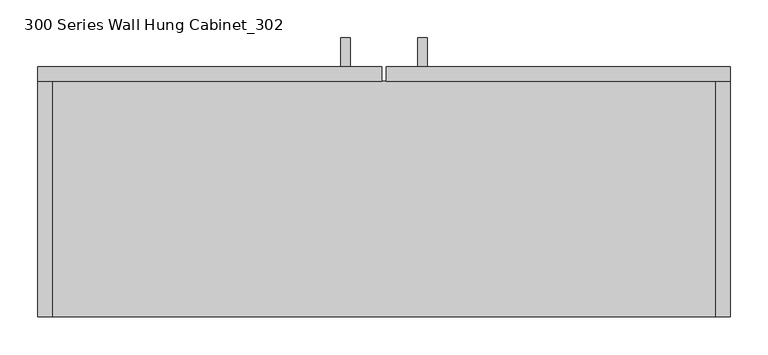
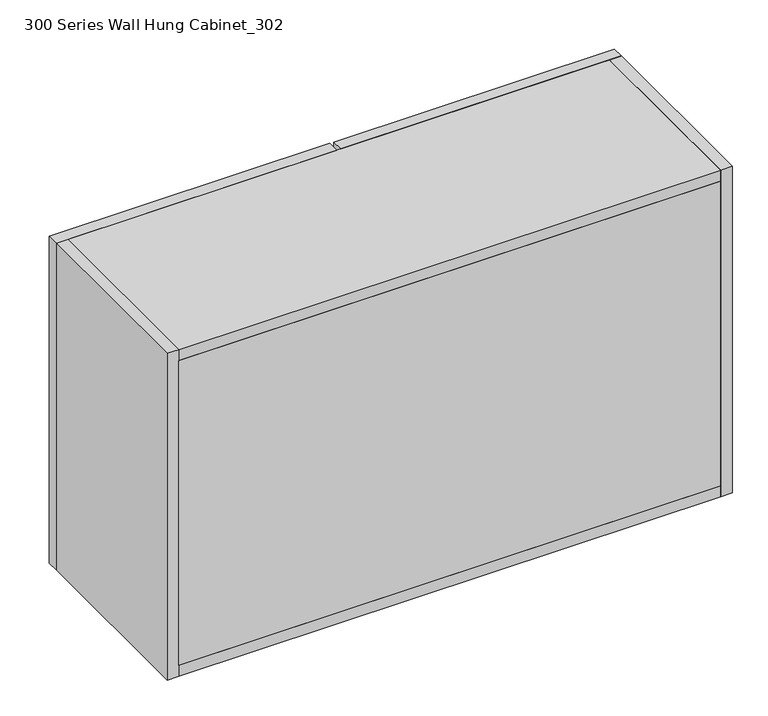
"""IFC4 building model written with IfcOpenShell, lengths in millimetres: furniture geometry, 300 Series Wall Hung Cabinet_302."""

import ifcopenshell
import ifcopenshell.guid

model = None  # the IFC model being written
_history = None  # IfcOwnerHistory: only IFC2X3 demands one
_inside = {}  # id of a spatial element -> (the spatial element, [elements in it])
_under = {}  # id of a project, library or spatial element -> (it, [spatial elements below it])
_declared = {}  # id of a project -> (the project, [libraries it declares])
_typed = {}  # id of a type object -> (the type object, [elements of that type])
_made_of = {}  # id of a material, layer set ... -> (it, [elements and type objects made of it])


def new_model(schema):
    """Start an empty IFC model of exactly this schema.

    Asked for "IFC4X3", IfcOpenShell would pick the latest addendum, in which some entities
    have other attributes; the version numbers below select the first issue.
    IFC2X3 requires an IfcOwnerHistory on every rooted entity: one is made here for all.
    """
    global model, _history
    if schema == "IFC4X3":
        model = ifcopenshell.file(schema_version=(4, 3, 0, 0))
    else:
        model = ifcopenshell.file(schema=schema)
    _inside.clear()
    _under.clear()
    _declared.clear()
    _typed.clear()
    _made_of.clear()
    _history = None
    if model.schema == "IFC2X3":
        org = make("IfcOrganization", Name="unknown")
        user = make(
            "IfcPersonAndOrganization",
            ThePerson=make("IfcPerson", FamilyName="unknown"),
            TheOrganization=org,
        )
        app = make(
            "IfcApplication",
            ApplicationDeveloper=org,
            Version="unknown",
            ApplicationFullName="unknown",
            ApplicationIdentifier="unknown",
        )
        _history = make(
            "IfcOwnerHistory",
            OwningUser=user,
            OwningApplication=app,
            ChangeAction="ADDED",
            CreationDate=0,
        )
    return model


def make(cls, **values):
    """One entity of the class cls with the attributes given. An attribute that is None is left unset."""
    return model.create_entity(
        cls, **{name: value for name, value in values.items() if value is not None}
    )


def rooted(cls, **values):
    """An entity with a GlobalId (a new one), such as an element, a storey or a relation."""
    return make(cls, GlobalId=ifcopenshell.guid.new(), OwnerHistory=_history, **values)


def si_unit(unit_type, name, prefix=None):
    """IfcSIUnit, for example si_unit("LENGTHUNIT", "METRE", prefix="MILLI")."""
    return make("IfcSIUnit", UnitType=unit_type, Prefix=prefix, Name=name)


def assignment(units):
    """IfcUnitAssignment: the units of a project."""
    return None if units is None else make("IfcUnitAssignment", Units=units)


def point(xyz):
    """IfcCartesianPoint."""
    return None if xyz is None else make("IfcCartesianPoint", Coordinates=xyz)


def direction(xyz):
    """IfcDirection."""
    return None if xyz is None else make("IfcDirection", DirectionRatios=xyz)


def frame(location, z_axis=None, x_axis=None):
    """IfcAxis2Placement3D, a coordinate frame: its origin and axes. An axis left out is left unset."""
    return make(
        "IfcAxis2Placement3D",
        Location=point(location),
        Axis=direction(z_axis),
        RefDirection=direction(x_axis),
    )


def origin():
    """The frame at (0, 0, 0) with its axes left unset."""
    return frame((0.0, 0.0, 0.0))


def place(relative_to, where):
    """IfcLocalPlacement: puts the frame where relative to a parent placement (None: the world)."""
    return make(
        "IfcLocalPlacement", PlacementRelTo=relative_to, RelativePlacement=where
    )


def context(
    kind, dimensions, precision=None, world=None, true_north=None, identifier=None
):
    """IfcGeometricRepresentationContext, for example the 3D "Model" context."""
    return make(
        "IfcGeometricRepresentationContext",
        ContextIdentifier=identifier,
        ContextType=kind,
        CoordinateSpaceDimension=dimensions,
        Precision=precision,
        WorldCoordinateSystem=world,
        TrueNorth=true_north,
    )


def project(units=None, contexts=None):
    """IfcProject with its units and contexts."""
    return rooted(
        "IfcProject",
        Name="project",
        RepresentationContexts=contexts,
        UnitsInContext=assignment(units),
    )


def spatial(cls, under=None, at=None, **own):
    """A site, building, storey or space (cls), placed at a placement, below another one or the project."""
    s = rooted(cls, ObjectPlacement=at, **own)
    if under is not None:
        _under.setdefault(under.id(), (under, []))[1].append(s)
    return s


def polyline(points):
    """IfcPolyline through the points."""
    return make("IfcPolyline", Points=[point(p) for p in points])


def outline(outer, holes=None, kind="AREA"):
    """IfcArbitraryClosedProfileDef: a profile drawn as a closed curve; with holes, ...WithVoids."""
    if holes is None:
        return make("IfcArbitraryClosedProfileDef", ProfileType=kind, OuterCurve=outer)
    return make(
        "IfcArbitraryProfileDefWithVoids",
        ProfileType=kind,
        OuterCurve=outer,
        InnerCurves=holes,
    )


def extrude(swept, where, along, depth):
    """IfcExtrudedAreaSolid: the profile swept, set in the frame where, extruded along a direction by depth."""
    return make(
        "IfcExtrudedAreaSolid",
        SweptArea=swept,
        Position=where,
        ExtrudedDirection=direction(along),
        Depth=depth,
    )


def shape(context_of_items, identifier, shape_type, items):
    """IfcShapeRepresentation: the items that make up one representation, for example the "Body"."""
    return make(
        "IfcShapeRepresentation",
        ContextOfItems=context_of_items,
        RepresentationIdentifier=identifier,
        RepresentationType=shape_type,
        Items=items,
    )


def source(mapping_origin, context_of_items, identifier, shape_type, items):
    """IfcRepresentationMap: a shape defined once, which mapped items show again and again."""
    return make(
        "IfcRepresentationMap",
        MappingOrigin=mapping_origin,
        MappedRepresentation=shape(context_of_items, identifier, shape_type, items),
    )


def transform(
    local_origin,
    x_axis=None,
    y_axis=None,
    z_axis=None,
    scale=None,
    scale2=None,
    scale3=None,
    uniform=True,
):
    """IfcCartesianTransformationOperator3D, or its non-uniform kind. x_axis, y_axis, z_axis: its Axis1, 2, 3."""
    if uniform:
        return make(
            "IfcCartesianTransformationOperator3D",
            Axis1=direction(x_axis),
            Axis2=direction(y_axis),
            LocalOrigin=point(local_origin),
            Scale=scale,
            Axis3=direction(z_axis),
        )
    return make(
        "IfcCartesianTransformationOperator3DnonUniform",
        Axis1=direction(x_axis),
        Axis2=direction(y_axis),
        LocalOrigin=point(local_origin),
        Scale=scale,
        Axis3=direction(z_axis),
        Scale2=scale2,
        Scale3=scale3,
    )


def mapped(mapping_source, mapping_target):
    """IfcMappedItem: shows the shape of a source again, moved by a transform."""
    return make(
        "IfcMappedItem", MappingSource=mapping_source, MappingTarget=mapping_target
    )


def made_of(thing, what):
    """Note that an element or type object is made of a material, layer set ...; save() writes the relation."""
    if what is not None:
        _made_of.setdefault(what.id(), (what, []))[1].append(thing)
    return thing


def element(
    cls,
    number,
    at=None,
    inside=None,
    cuts=None,
    type_object=None,
    material=None,
    context=None,
    identifier="Body",
    shape_type=None,
    held_by="IfcProductDefinitionShape",
    body=None,
    shapes=None,
    **own,
):
    """One element of the class cls, such as IfcWall. Its Tag is "e" and its number.

    at: its placement. inside: the storey or other place that contains it. cuts: it is an
    opening in that element (IfcRelVoidsElement). A single representation is given by context,
    identifier, shape_type and body (its items); several are given by shapes. held_by: the class
    of the entity that holds the representations. save() writes the other relations.
    """
    e = rooted(cls, Tag="e%d" % number, ObjectPlacement=at, **own)
    if body is not None:
        shapes = [shape(context, identifier, shape_type, body)]
    if shapes is not None:
        e.Representation = make(held_by, Representations=shapes)
    if inside is not None:
        _inside.setdefault(inside.id(), (inside, []))[1].append(e)
    if cuts is not None:
        rooted(
            "IfcRelVoidsElement", RelatingBuildingElement=cuts, RelatedOpeningElement=e
        )
    if type_object is not None:
        _typed.setdefault(type_object.id(), (type_object, []))[1].append(e)
    return made_of(e, material)


def aggregate(whole, parts):
    """IfcRelAggregates: a whole, such as a stair, and the parts it consists of."""
    return rooted("IfcRelAggregates", RelatingObject=whole, RelatedObjects=parts)


def save(model, path):
    """Write the relations noted so far, then the file.

    IfcRelAggregates (storeys below a building ...), IfcRelContainedInSpatialStructure (elements
    in a storey), IfcRelDefinesByType, IfcRelAssociatesMaterial and IfcRelDeclares: one each for
    every whole, place, type object, material and project.
    """
    for whole, parts in _under.values():
        aggregate(whole, parts)
    for where, things in _inside.values():
        rooted(
            "IfcRelContainedInSpatialStructure",
            RelatedElements=things,
            RelatingStructure=where,
        )
    for kind, things in _typed.values():
        rooted("IfcRelDefinesByType", RelatedObjects=things, RelatingType=kind)
    for what, things in _made_of.values():
        rooted("IfcRelAssociatesMaterial", RelatedObjects=things, RelatingMaterial=what)
    for by, libraries in _declared.values():
        rooted("IfcRelDeclares", RelatingContext=by, RelatedDefinitions=libraries)
    model.write(path)


def furniture_300_series_wall_hung_cabinet_302_8891d94a(model_context):
    return source(origin(), model_context, "Body", "SweptSolid", [
        extrude(outline(polyline([(390.525, 1708.1425373), (390.525, 1720.8121874), (428.6060937, 1720.8121874), (428.6060937, 1625.6), (390.525, 1625.6), (390.525, 1638.2696501), (415.9364436, 1638.2696501), (415.9364436, 1708.1425373), (390.525, 1708.1425373)])), frame((-57.15, 0.0, 0.0), z_axis=(1.0, 0.0, 0.0), x_axis=(0.0, 1.0, 0.0)), (0.0, 0.0, 1.0), 12.4065288),
        extrude(outline(polyline([(390.525, 1708.1425373), (390.525, 1720.8121874), (428.6060937, 1720.8121874), (428.6060937, 1625.6), (390.525, 1625.6), (390.525, 1638.2696501), (415.9364436, 1638.2696501), (415.9364436, 1708.1425373), (390.525, 1708.1425373)])), frame((44.45, 0.0, 0.0), z_axis=(1.0, 0.0, 0.0), x_axis=(0.0, 1.0, 0.0)), (0.0, 0.0, 1.0), 12.4065288),
        extrude(outline(polyline([(438.15, 60.325), (-438.15, 60.325), (-438.15, 79.375), (438.15, 79.375), (438.15, 60.325)])), frame((0.0, 0.0, 1593.85), z_axis=(0.0, 0.0, 1.0), x_axis=(1.0, 0.0, 0.0)), (0.0, 0.0, 1.0), 520.7),
        extrude(outline(polyline([(-3.175, 371.475), (-457.2, 371.475), (-457.2, 390.525), (-3.175, 390.525), (-3.175, 371.475)])), frame((0.0, 0.0, 1574.8), z_axis=(0.0, 0.0, 1.0), x_axis=(1.0, 0.0, 0.0)), (0.0, 0.0, 1.0), 558.8),
        extrude(outline(polyline([(457.2, 371.475), (3.175, 371.475), (3.175, 390.525), (457.2, 390.525), (457.2, 371.475)])), frame((0.0, 0.0, 1574.8), z_axis=(0.0, 0.0, 1.0), x_axis=(1.0, 0.0, 0.0)), (0.0, 0.0, 1.0), 558.8),
        extrude(outline(polyline([(-457.2, 60.325), (-457.2, 371.475), (-438.15, 371.475), (-438.15, 60.325), (-457.2, 60.325)])), frame((0.0, 0.0, 1574.8), z_axis=(0.0, 0.0, 1.0), x_axis=(1.0, 0.0, 0.0)), (0.0, 0.0, 1.0), 558.8),
        extrude(outline(polyline([(438.15, 60.325), (438.15, 371.475), (457.2, 371.475), (457.2, 60.325), (438.15, 60.325)])), frame((0.0, 0.0, 1574.8), z_axis=(0.0, 0.0, 1.0), x_axis=(1.0, 0.0, 0.0)), (0.0, 0.0, 1.0), 558.8),
        extrude(outline(polyline([(438.15, 371.475), (438.15, 60.325), (-438.15, 60.325), (-438.15, 371.475), (438.15, 371.475)])), frame((0.0, 0.0, 2114.55), z_axis=(0.0, 0.0, 1.0), x_axis=(1.0, 0.0, 0.0)), (0.0, 0.0, 1.0), 19.05),
        extrude(outline(polyline([(438.15, 371.475), (438.15, 60.325), (-438.15, 60.325), (-438.15, 371.475), (438.15, 371.475)])), frame((0.0, 0.0, 1574.8), z_axis=(0.0, 0.0, 1.0), x_axis=(1.0, 0.0, 0.0)), (0.0, 0.0, 1.0), 19.05),
    ])


if __name__ == "__main__":
    model = new_model("IFC4")
    model_context = context("Model", 3, world=origin())
    ifc_project = project(units=[si_unit("LENGTHUNIT", "METRE", prefix="MILLI")], contexts=[model_context])
    site = spatial("IfcSite", under=ifc_project)
    building = spatial("IfcBuilding", under=site)
    placement = place(None, origin())
    furniture_300_series_wall_hung_cabinet_302_shape = furniture_300_series_wall_hung_cabinet_302_8891d94a(model_context)
    element("IfcFurniture", 1, ObjectType="300 Series Wall Hung Cabinet_302 : 36\"W x 21\"H", at=placement, inside=building, context=model_context, shape_type="MappedRepresentation", body=[
        mapped(furniture_300_series_wall_hung_cabinet_302_shape, transform((0.0, 0.0, 0.0), x_axis=(1.0, 0.0, 0.0), y_axis=(0.0, 1.0, 0.0), z_axis=(0.0, 0.0, 1.0))),
    ])
    save(model, "model.ifc")

# Revit data of these elements
# Type "300 Series Wall Hung Cabinet_302 : 36\"W x 21\"H"
#   URL = "www.wicnet.org/manual_sections.asp"
#   Model = "302"
#   Manufacturer = "Woodwork Institute"
#   Description = "Wall Hung Cabinet"
#   Content Creator URL = "www.AECcontent.com"
#   Content Creator = "AECcontent"
#   Assembly Code = "E2010200"
#   Width = 3' - 0"
#   Top of Cabinet = 7' - 0"
#   Height = 1' - 10"
#   Depth = 1' - 1"
#   Top Panel Material = none
#   Side Panel Material = none
#   Shelf Panel Material = none
#   Door Panel Material = none
# Element 1 (IfcFurniture, "300 Series Wall Hung Cabinet_302 : 36\"W x 21\"H")
#   Materials on its faces: "CASEWORK"
# Materials
#   "CASEWORK": class "Generic", colour RGB 181 181 181, transparency 0, Cost = 0
